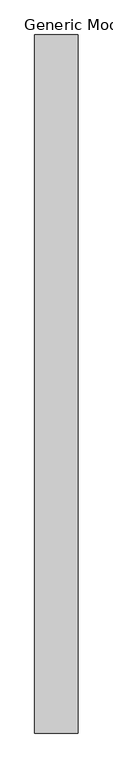
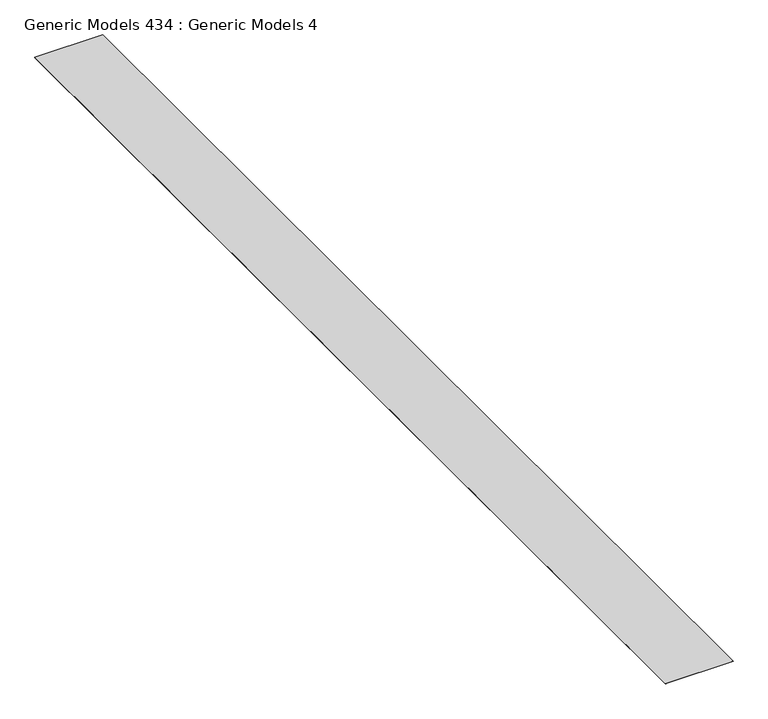
"""IFC4 building model written with IfcOpenShell, lengths in millimetres: proxy geometry, Generic Models 434 : Generic Models 4."""

from ifc_helpers import new_model, si_unit, frame, origin, place, context, project, spatial, polyline, outline, extrude, source, transform, mapped, element, save


def generic_models_434_generic_models_4_b5b4e9ea(model_context):
    return source(origin(), model_context, "Body", "SweptSolid", [
        extrude(outline(polyline([(8394.5263704, -5493.3230338), (7905.5763704, -5493.3230338), (7905.5763704, 2393.3769662), (8394.5263704, 2393.3769662), (8394.5263704, -5493.3230338)])), frame((0.0, 0.0, 123550.1085), z_axis=(0.0, 0.0, 1.0), x_axis=(1.0, 0.0, 0.0)), (0.0, 0.0, 1.0), 1.5875),
    ])


if __name__ == "__main__":
    model = new_model("IFC4")
    model_context = context("Model", 3, world=origin())
    ifc_project = project(units=[si_unit("LENGTHUNIT", "METRE", prefix="MILLI")], contexts=[model_context])
    site = spatial("IfcSite", under=ifc_project)
    building = spatial("IfcBuilding", under=site)
    placement = place(None, origin())
    generic_models_434_generic_models_4_shape = generic_models_434_generic_models_4_b5b4e9ea(model_context)
    element("IfcBuildingElementProxy", 1, Name="Generic Models 434 : Generic Models 4", ObjectType="Generic Models 434 : Generic Models 4", at=placement, inside=building, context=model_context, shape_type="MappedRepresentation", body=[
        mapped(generic_models_434_generic_models_4_shape, transform((0.0, 0.0, 0.0), x_axis=(1.0, 0.0, 0.0), y_axis=(0.0, 1.0, 0.0), z_axis=(0.0, 0.0, 1.0))),
    ])
    save(model, "model.ifc")

# Revit data of these elements
# Element 1 (IfcBuildingElementProxy, "Generic Models 434 : Generic Models 4")
#   Materials on its faces: "_15 MIL VAPOR BARRIER"
# Materials
#   "_15 MIL VAPOR BARRIER": class "Generic", colour RGB 67 154 161, transparency 0, Cost = 0
